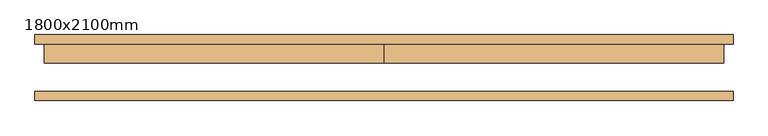
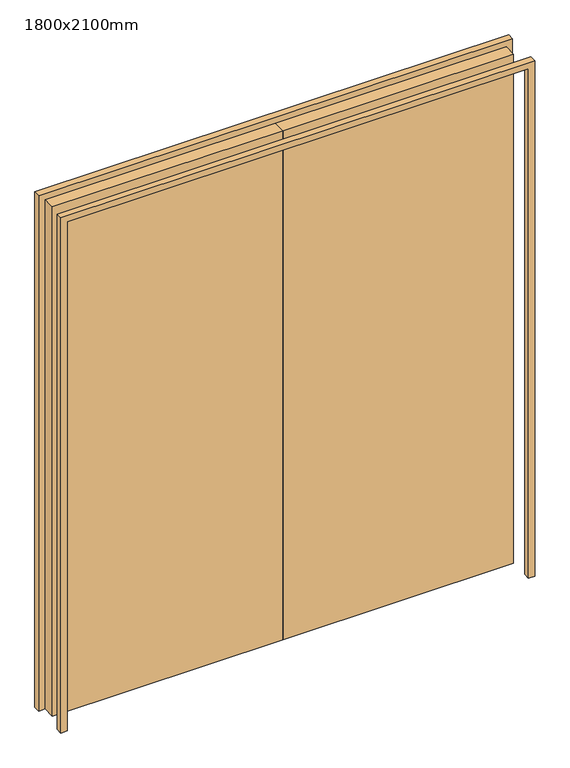
"""IFC4 building model written with IfcOpenShell, lengths in millimetres: door geometry, WWm-DoubleSolid-Flush : 1800x2100mm."""

from ifc_helpers import new_model, si_unit, frame, origin, origin_with_axes, place, context, project, spatial, polyline, outline, extrude, source, transform, mapped, element, save


def door_1800x2100mm_7a34d599(model_context):
    return source(origin(), model_context, "Body", "SweptSolid", [
        extrude(outline(polyline([(0.0, 62.5), (900.0, 62.5), (900.0, 12.5), (0.0, 12.5), (0.0, 62.5)])), origin_with_axes(), (0.0, 0.0, 1.0), 2100.0),
        extrude(outline(polyline([(-900.0, 62.5), (0.0, 62.5), (0.0, 12.5), (-900.0, 12.5), (-900.0, 62.5)])), origin_with_axes(), (0.0, 0.0, 1.0), 2100.0),
        extrude(outline(polyline([(2100.0, -900.0), (2100.0, 900.0), (0.0, 900.0), (0.0, 925.0), (2125.0, 925.0), (2125.0, -925.0), (0.0, -925.0), (0.0, -900.0), (2100.0, -900.0)])), frame((0.0, -87.5, 0.0), z_axis=(0.0, 1.0, 0.0), x_axis=(0.0, 0.0, 1.0)), (0.0, 0.0, 1.0), 25.0),
        extrude(outline(polyline([(2100.0, -900.0), (2100.0, 900.0), (0.0, 900.0), (0.0, 925.0), (2125.0, 925.0), (2125.0, -925.0), (0.0, -925.0), (0.0, -900.0), (2100.0, -900.0)])), frame((0.0, 62.5, 0.0), z_axis=(0.0, 1.0, 0.0), x_axis=(0.0, 0.0, 1.0)), (0.0, 0.0, 1.0), 25.0),
    ])


if __name__ == "__main__":
    model = new_model("IFC4")
    model_context = context("Model", 3, world=origin())
    ifc_project = project(units=[si_unit("LENGTHUNIT", "METRE", prefix="MILLI")], contexts=[model_context])
    site = spatial("IfcSite", under=ifc_project)
    building = spatial("IfcBuilding", under=site)
    placement = place(None, origin())
    door_1800x2100mm_shape = door_1800x2100mm_7a34d599(model_context)
    element("IfcDoor", 1, ObjectType="WWm-DoubleSolid-Flush : 1800x2100mm", at=placement, inside=building, context=model_context, shape_type="MappedRepresentation", body=[
        mapped(door_1800x2100mm_shape, transform((0.0, 0.0, 0.0), x_axis=(1.0, 0.0, 0.0), y_axis=(0.0, 1.0, 0.0), z_axis=(0.0, 0.0, 1.0))),
    ])
    save(model, "model.ifc")

# Revit data of these elements
# Type "WWm-DoubleSolid-Flush : 1800x2100mm"
#   Type Mark = "EX1-44"
#   Construction Type Id = "MDOOR"
#   Assembly Code = "C1020"
#   Analytic Construction = "Metal"
#   Thickness = 50 mm
#   Thermal Resistance (R) = 0.270117 (m²·K)/W
#   Heat Transfer Coefficient (U) = 3.7021 W/(m²·K)
#   Height = 2100 mm
#   Trim Projection Ext = 25 mm
#   Trim Projection Int = 25 mm
#   Trim Width = 25 mm
#   Width = 1800 mm
#   Not 90 Degree [instance default] = no
#   90 Degree [instance default] = yes
#   Door Material = WW-EC-RGB-White
#   Frame Material = WW-EC-RGB-White
#   Visual Light Transmittance = 0
#   Solar Heat Gain Coefficient = 0
#   Function = (empty or 0)
#   Wall Closure = (empty or 0)
# Element 1 (IfcDoor, "WWm-DoubleSolid-Flush : 1800x2100mm")
#   Materials on its faces: "WW-EC-RGB-White"
# Materials
#   "WW-EC-RGB-White": class "Generic", colour RGB 255 255 255, transparency 0, Comments = "If region requests off-white, swith asset color to RGB 231-228-220", Description = "Generic Color", Cost = 0
